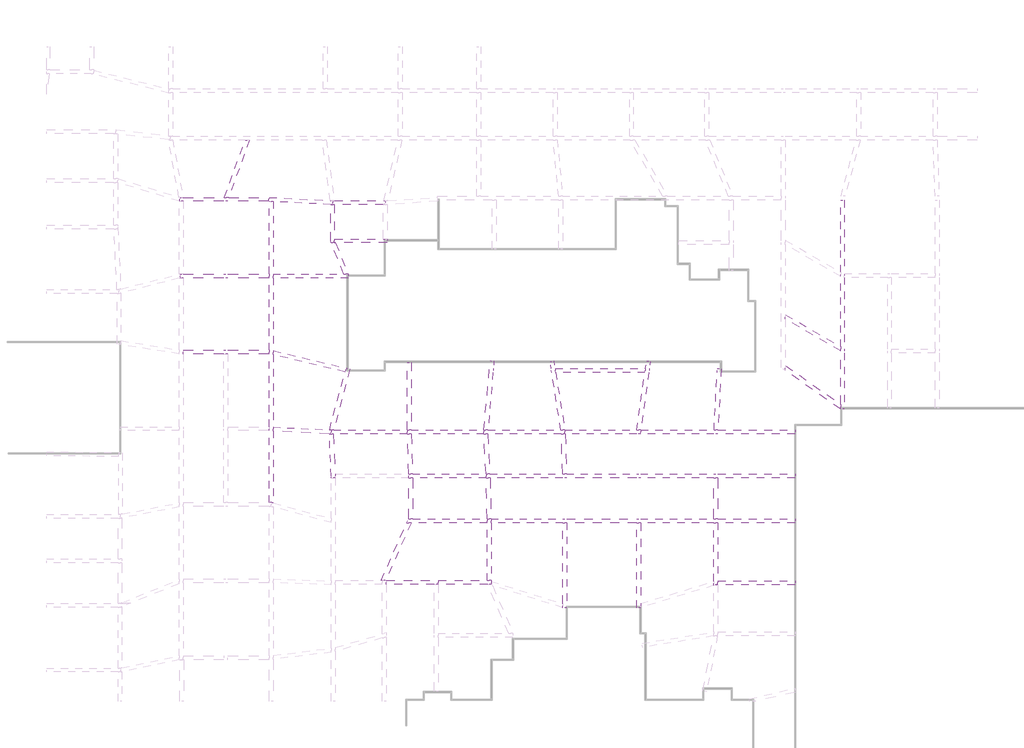
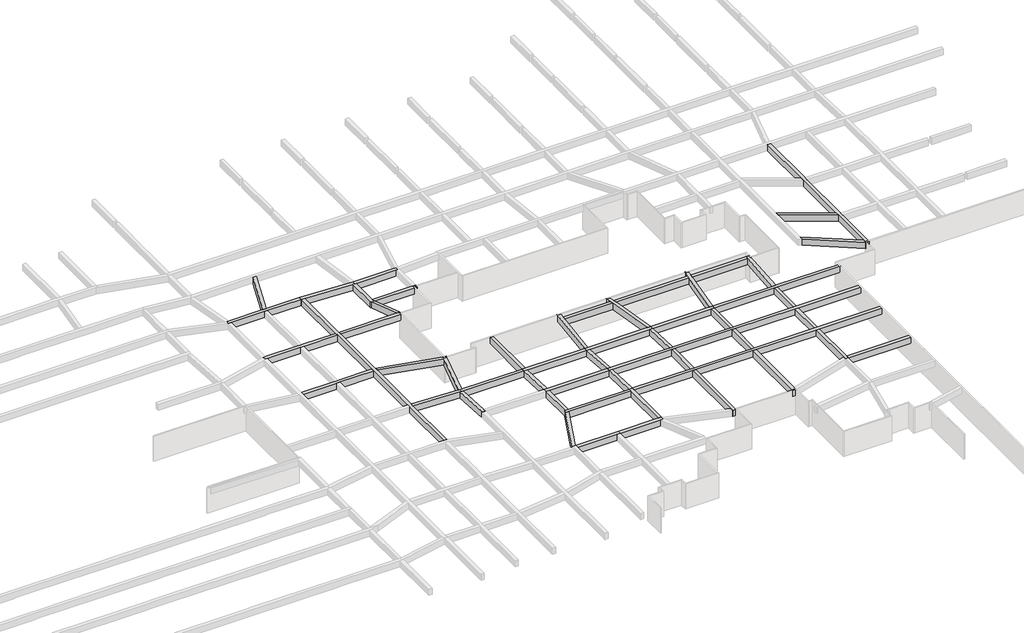
# One storey, part 17 of 45: 47 beams.
"""IFC4 building model written with IfcOpenShell, lengths in millimetres."""

from ifc_helpers import new_model, si_unit, frame, origin, place, context, project, spatial, polyline, outline, extrude, faceted_brep, element, save

model = new_model("IFC4")

# Units and contexts
model_context = context("Model", 3, world=origin())
ifc_project = project(units=[si_unit("LENGTHUNIT", "METRE", prefix="MILLI")], contexts=[model_context])

# Site, building, storey
site = spatial("IfcSite", under=ifc_project)
building = spatial("IfcBuilding", under=site)
storey = spatial("IfcBuildingStorey", under=building, Name="户型图", Elevation=0.0)

# Beams
placement = place(None, origin())
element("IfcBeam", 1, ObjectType="混凝土 - 矩形梁 : KL_beam", at=placement, inside=storey, context=model_context, shape_type="Brep", body=[
    faceted_brep([(-58675.077, -88790.3844516, 3300.0), (-58664.6026314, -88390.3844516, 3300.0), (-62792.0400184, -88390.3844516, 3300.0), (-63217.7111274, -88390.3844516, 3300.0), (-67462.9624722, -88390.3844516, 3300.0), (-67740.4118212, -88390.3844516, 3300.0), (-67799.2678102, -88790.3844516, 3300.0), (-67430.7823984, -88790.3844516, 3300.0), (-63277.6696197, -88790.3844516, 3300.0), (-62877.6696197, -88790.3844516, 3300.0), (-58675.077, -88790.3844516, 2500.0), (-67799.2678102, -88790.3844516, 2500.0), (-67430.7823984, -88790.3844516, 2500.0), (-63277.6696197, -88790.3844516, 2500.0), (-62877.6696197, -88790.3844516, 2500.0), (-58664.6026314, -88390.3844516, 2500.0), (-67740.4118212, -88390.3844516, 2500.0), (-67462.9624722, -88390.3844516, 2500.0), (-63217.7111274, -88390.3844516, 2500.0), (-62792.0400184, -88390.3844516, 2500.0)], [[[0, 1, 2, 3, 4, 5, 6, 7, 8, 9]], [[10, 0, 9, 8, 7, 6, 11, 12, 13, 14]], [[15, 10, 14, 13, 12, 11, 16, 17, 18, 19]], [[1, 15, 19, 18, 17, 16, 5, 4, 3, 2]], [[5, 16, 11, 6]], [[1, 0, 10, 15]]]),
])
element("IfcBeam", 2, ObjectType="混凝土 - 矩形梁 : KL_beam", at=placement, inside=storey, context=model_context, shape_type="Brep", body=[
    faceted_brep([(-67725.9320986, -96211.286122, 3300.0), (-67675.9190824, -96611.286122, 3300.0), (-67430.7823984, -96611.286122, 3300.0), (-63277.6696197, -96611.286122, 3300.0), (-62877.6696197, -96611.286122, 3300.0), (-58630.7823984, -96611.286122, 3300.0), (-58630.7823984, -96211.286122, 3300.0), (-62877.6696197, -96211.286122, 3300.0), (-63277.6696197, -96211.286122, 3300.0), (-67430.7823984, -96211.286122, 3300.0), (-67675.9190824, -96611.286122, 2500.0), (-67430.7823984, -96611.286122, 2500.0), (-63277.6696197, -96611.286122, 2500.0), (-62877.6696197, -96611.286122, 2500.0), (-58630.7823984, -96611.286122, 2500.0), (-67725.9320986, -96211.286122, 2500.0), (-67430.7823984, -96211.286122, 2500.0), (-63277.6696197, -96211.286122, 2500.0), (-62877.6696197, -96211.286122, 2500.0), (-58630.7823984, -96211.286122, 2500.0)], [[[0, 1, 2, 3, 4, 5, 6, 7, 8, 9]], [[1, 10, 11, 12, 13, 14, 5, 4, 3, 2]], [[10, 15, 16, 17, 18, 19, 14, 13, 12, 11]], [[15, 0, 9, 8, 7, 6, 19, 18, 17, 16]], [[0, 15, 10, 1]], [[6, 5, 14, 19]]]),
])
element("IfcBeam", 3, ObjectType="混凝土 - 矩形梁 : KL_beam", at=placement, inside=storey, context=model_context, shape_type="Brep", body=[
    faceted_brep([(-52173.5106555, -88730.5681671, 3300.0), (-52408.1333935, -88718.2721105, 3300.0), (-58664.6026314, -88390.3844516, 3300.0), (-58675.077, -88790.3844516, 3300.0), (-58630.7823984, -88792.7058333, 3300.0), (-58230.7823984, -88813.668945, 3300.0), (-52378.7478398, -89120.3610805, 3300.0), (-52183.9850241, -89130.5681671, 3300.0), (-58675.077, -88790.3844516, 2500.0), (-58630.7823984, -88792.7058333, 2500.0), (-58230.7823984, -88813.668945, 2500.0), (-52378.7478398, -89120.3610805, 2500.0), (-52183.9850241, -89130.5681671, 2500.0), (-58664.6026314, -88390.3844516, 2500.0), (-52408.1333935, -88718.2721105, 2500.0), (-52173.5106555, -88730.5681671, 2500.0)], [[[0, 1, 2, 3, 4, 5, 6, 7]], [[7, 6, 5, 4, 3, 8, 9, 10, 11, 12]], [[12, 11, 10, 9, 8, 13, 14, 15]], [[2, 1, 0, 15, 14, 13]], [[2, 13, 8, 3]], [[0, 7, 12, 15]]]),
])
element("IfcBeam", 4, ObjectType="混凝土 - 矩形梁 : KL_beam", at=placement, inside=storey, context=model_context, shape_type="Brep", body=[
    faceted_brep([(-46785.1341431, -88730.5681671, 3300.0), (-46937.8350231, -88730.5681671, 3300.0), (-52003.1410987, -88730.5681671, 3300.0), (-52173.5106555, -88730.5681671, 3300.0), (-52183.9850241, -89130.5681671, 3300.0), (-51978.7478398, -89130.5681671, 3300.0), (-46978.6472042, -89130.5681671, 3300.0), (-46772.3615365, -89130.5681671, 3300.0), (-52183.9850241, -89130.5681671, 2500.0), (-51978.7478398, -89130.5681671, 2500.0), (-46978.6472042, -89130.5681671, 2500.0), (-46772.3615365, -89130.5681671, 2500.0), (-52173.5106555, -88730.5681671, 2500.0), (-52003.1410987, -88730.5681671, 2500.0), (-46937.8350231, -88730.5681671, 2500.0), (-46785.1341431, -88730.5681671, 2500.0)], [[[0, 1, 2, 3, 4, 5, 6, 7]], [[7, 6, 5, 4, 8, 9, 10, 11]], [[11, 10, 9, 8, 12, 13, 14, 15]], [[3, 2, 1, 0, 15, 14, 13, 12]], [[3, 12, 8, 4]], [[0, 7, 11, 15]]]),
])
element("IfcBeam", 5, ObjectType="混凝土 - 矩形梁 : KL_beam", at=placement, inside=storey, context=model_context, shape_type="Brep", body=[
    faceted_brep([(-51978.7478398, -89130.5681671, 3300.0), (-52183.9850241, -89130.5681671, 3300.0), (-52355.5272319, -89121.578021, 3300.0), (-52378.7478398, -89120.3610805, 3300.0), (-52378.7478398, -92869.4623087, 3300.0), (-52313.6241975, -93030.5681671, 3300.0), (-51978.7478398, -93030.5681671, 3300.0), (-51978.7478398, -92630.5681671, 3300.0), (-52378.7478398, -89120.3610805, 2500.0), (-52378.7478398, -92869.4623087, 2500.0), (-52183.9850241, -89130.5681671, 2500.0), (-51978.7478398, -89130.5681671, 2500.0), (-51978.7478398, -92630.5681671, 2500.0), (-51978.7478398, -93030.5681671, 2500.0), (-52313.6241975, -93030.5681671, 2500.0), (-52355.5272319, -89121.578021, 2500.0)], [[[0, 1, 2, 3, 4, 5, 6, 7]], [[3, 8, 9, 4]], [[10, 11, 12, 13, 14, 9, 8, 15]], [[11, 0, 7, 6, 13, 12]], [[8, 3, 2, 1, 10, 15]], [[1, 0, 11, 10]], [[6, 5, 14, 13]], [[14, 5, 4, 9]]]),
])
element("IfcBeam", 6, ObjectType="混凝土 - 矩形梁 : KL_beam", at=placement, inside=storey, context=model_context, shape_type="Brep", body=[
    faceted_brep([(-46578.6472042, -93030.5681671, 3300.0), (-46578.6472042, -92630.5681671, 3300.0), (-46978.6472042, -92630.5681671, 3300.0), (-51978.7478398, -92630.5681671, 3300.0), (-51978.7478398, -93030.5681671, 3300.0), (-51882.1799262, -93030.5681671, 3300.0), (-46578.6472042, -93030.5681671, 2500.0), (-51978.7478398, -93030.5681671, 2500.0), (-51882.1799262, -93030.5681671, 2500.0), (-46578.6472042, -92630.5681671, 2500.0), (-51978.7478398, -92630.5681671, 2500.0), (-46978.6472042, -92630.5681671, 2500.0)], [[[0, 1, 2, 3, 4, 5]], [[6, 0, 5, 4, 7, 8]], [[9, 6, 8, 7, 10, 11]], [[1, 9, 11, 10, 3, 2]], [[4, 3, 10, 7]], [[1, 0, 6, 9]]]),
])
element("IfcBeam", 7, ObjectType="混凝土 - 矩形梁 : KL_beam", at=placement, inside=storey, context=model_context, shape_type="Brep", body=[
    faceted_brep([(-41387.6738698, -127942.8806028, 3300.0), (-41387.6738698, -127542.8806028, 3300.0), (-46687.6738698, -127542.8806028, 3300.0), (-46687.6738698, -127942.8806028, 3300.0), (-41787.6738698, -127942.8806028, 3300.0), (-41387.6738698, -127942.8806028, 2500.0), (-46687.6738698, -127942.8806028, 2500.0), (-41787.6738698, -127942.8806028, 2500.0), (-41387.6738698, -127542.8806028, 2500.0), (-46687.6738698, -127542.8806028, 2500.0)], [[[0, 1, 2, 3, 4]], [[5, 0, 4, 3, 6, 7]], [[8, 5, 7, 6, 9]], [[1, 8, 9, 2]], [[3, 2, 9, 6]], [[1, 0, 5, 8]]]),
])
element("IfcBeam", 8, ObjectType="混凝土 - 矩形梁 : KL_beam", at=placement, inside=storey, context=model_context, shape_type="Brep", body=[
    faceted_brep([(-35987.6738698, -127942.8806028, 3300.0), (-35987.6738698, -127702.1901429, 3300.0), (-35987.6738698, -127596.1274566, 3300.0), (-35987.6738698, -127542.8806028, 3300.0), (-36387.6738698, -127542.8806028, 3300.0), (-41387.6738698, -127542.8806028, 3300.0), (-41387.6738698, -127942.8806028, 3300.0), (-36320.0509821, -127942.8806028, 3300.0), (-35987.6738698, -127942.8806028, 2500.0), (-41387.6738698, -127942.8806028, 2500.0), (-36320.0509821, -127942.8806028, 2500.0), (-35987.6738698, -127542.8806028, 2500.0), (-35987.6738698, -127596.1274566, 2500.0), (-35987.6738698, -127702.1901429, 2500.0), (-41387.6738698, -127542.8806028, 2500.0), (-36387.6738698, -127542.8806028, 2500.0)], [[[0, 1, 2, 3, 4, 5, 6, 7]], [[8, 0, 7, 6, 9, 10]], [[11, 12, 13, 8, 10, 9, 14, 15]], [[3, 11, 15, 14, 5, 4]], [[3, 2, 1, 0, 8, 13, 12, 11]], [[6, 5, 14, 9]]]),
])
element("IfcBeam", 9, ObjectType="混凝土 - 矩形梁 : KL_beam", at=placement, inside=storey, context=model_context, shape_type="Brep", body=[
    faceted_brep([(-35987.6738698, -121242.8806028, 3300.0), (-35992.3975259, -121242.8806028, 3300.0), (-36387.6738698, -121242.8806028, 3300.0), (-36387.6738698, -121642.8806028, 3300.0), (-36387.6738698, -127542.8806028, 3300.0), (-35987.6738698, -127542.8806028, 3300.0), (-35987.6738698, -121642.8806028, 3300.0), (-35987.6738698, -121242.8806028, 2500.0), (-35987.6738698, -127542.8806028, 2500.0), (-35987.6738698, -121642.8806028, 2500.0), (-36387.6738698, -121242.8806028, 2500.0), (-35992.3975259, -121242.8806028, 2500.0), (-36387.6738698, -127542.8806028, 2500.0), (-36387.6738698, -121642.8806028, 2500.0)], [[[0, 1, 2, 3, 4, 5, 6]], [[7, 0, 6, 5, 8, 9]], [[10, 11, 7, 9, 8, 12, 13]], [[2, 10, 13, 12, 4, 3]], [[5, 4, 12, 8]], [[2, 1, 0, 7, 11, 10]]]),
])
element("IfcBeam", 10, ObjectType="混凝土 - 矩形梁 : KL_beam", at=placement, inside=storey, context=model_context, shape_type="Brep", body=[
    faceted_brep([(-44417.5553885, -121242.8806028, 3300.0), (-44595.6468626, -121642.8806028, 3300.0), (-44157.7923512, -121642.8806028, 3300.0), (-36387.6738698, -121642.8806028, 3300.0), (-36387.6738698, -121242.8806028, 3300.0), (-36392.5117893, -121242.8806028, 3300.0), (-43992.4702803, -121242.8806028, 3300.0), (-44392.4702803, -121242.8806028, 3300.0), (-44417.5553885, -121242.8806028, 2500.0), (-36387.6738698, -121242.8806028, 2500.0), (-36392.5117893, -121242.8806028, 2500.0), (-43992.4702803, -121242.8806028, 2500.0), (-44392.4702803, -121242.8806028, 2500.0), (-44595.6468626, -121642.8806028, 2500.0), (-36387.6738698, -121642.8806028, 2500.0), (-44157.7923512, -121642.8806028, 2500.0)], [[[0, 1, 2, 3, 4, 5, 6, 7]], [[8, 0, 7, 6, 5, 4, 9, 10, 11, 12]], [[13, 8, 12, 11, 10, 9, 14, 15]], [[1, 13, 15, 14, 3, 2]], [[4, 3, 14, 9]], [[1, 0, 8, 13]]]),
])
element("IfcBeam", 11, ObjectType="混凝土 - 矩形梁 : KL_beam", at=placement, inside=storey, context=model_context, shape_type="Brep", body=[
    faceted_brep([(-44157.7923512, -121642.8806028, 3300.0), (-44595.6468626, -121642.8806028, 3300.0), (-47222.4961059, -127542.8806028, 3300.0), (-47087.6738698, -127542.8806028, 3300.0), (-46784.6415945, -127542.8806028, 3300.0), (-44595.6468626, -121642.8806028, 2500.0), (-47222.4961059, -127542.8806028, 2500.0), (-44157.7923512, -121642.8806028, 2500.0), (-46784.6415945, -127542.8806028, 2500.0), (-47087.6738698, -127542.8806028, 2500.0)], [[[0, 1, 2, 3, 4]], [[1, 5, 6, 2]], [[5, 7, 8, 9, 6]], [[7, 0, 4, 8]], [[1, 0, 7, 5]], [[4, 3, 2, 6, 9, 8]]]),
])
element("IfcBeam", 12, ObjectType="混凝土 - 矩形梁 : KL_beam", at=placement, inside=storey, context=model_context, shape_type="Brep", body=[
    faceted_brep([(-4940.5977631, -121242.8806028, 3300.0), (-4940.5977631, -121642.8806028, 3300.0), (-4940.5977631, -121642.8806028, 2500.0), (-4940.5977631, -121242.8806028, 2500.0), (-12840.9657871, -121242.8806028, 3300.0), (-13240.9657871, -121242.8806028, 3300.0), (-20732.9657871, -121242.8806028, 3300.0), (-21132.9657871, -121242.8806028, 3300.0), (-28276.0008118, -121242.8806028, 3300.0), (-28676.0008118, -121242.8806028, 3300.0), (-35987.6738698, -121242.8806028, 3300.0), (-35987.6738698, -121642.8806028, 3300.0), (-28676.0008118, -121642.8806028, 3300.0), (-28276.0008118, -121642.8806028, 3300.0), (-21132.9657871, -121642.8806028, 3300.0), (-20732.9657871, -121642.8806028, 3300.0), (-13240.9657871, -121642.8806028, 3300.0), (-12840.9657871, -121642.8806028, 3300.0), (-35987.6738698, -121642.8806028, 2500.0), (-28676.0008118, -121642.8806028, 2500.0), (-28276.0008118, -121642.8806028, 2500.0), (-21132.9657871, -121642.8806028, 2500.0), (-20732.9657871, -121642.8806028, 2500.0), (-13240.9657871, -121642.8806028, 2500.0), (-12840.9657871, -121642.8806028, 2500.0), (-35987.6738698, -121242.8806028, 2500.0), (-28676.0008118, -121242.8806028, 2500.0), (-28276.0008118, -121242.8806028, 2500.0), (-21132.9657871, -121242.8806028, 2500.0), (-20732.9657871, -121242.8806028, 2500.0), (-13240.9657871, -121242.8806028, 2500.0), (-12840.9657871, -121242.8806028, 2500.0)], [[[0, 1, 2, 3]], [[1, 0, 4, 5, 6, 7, 8, 9, 10, 11, 12, 13, 14, 15, 16, 17]], [[2, 1, 17, 16, 15, 14, 13, 12, 11, 18, 19, 20, 21, 22, 23, 24]], [[3, 2, 24, 23, 22, 21, 20, 19, 18, 25, 26, 27, 28, 29, 30, 31]], [[0, 3, 31, 30, 29, 28, 27, 26, 25, 10, 9, 8, 7, 6, 5, 4]], [[11, 10, 25, 18]]]),
])
element("IfcBeam", 13, ObjectType="混凝土 - 矩形梁 : KL_beam", at=placement, inside=storey, context=model_context, shape_type="Brep", body=[
    faceted_brep([(-28462.3909606, -112558.1512167, 3300.0), (-28462.3909606, -112158.1512167, 3300.0), (-28867.3770109, -112158.1512167, 3300.0), (-36315.5397573, -112158.1512167, 3300.0), (-36717.0676923, -112158.1512167, 3300.0), (-36717.0676923, -112558.1512167, 3300.0), (-36322.6397923, -112558.1512167, 3300.0), (-28826.6420326, -112558.1512167, 3300.0), (-28462.3909606, -112558.1512167, 2500.0), (-36717.0676923, -112558.1512167, 2500.0), (-36322.6397923, -112558.1512167, 2500.0), (-28826.6420326, -112558.1512167, 2500.0), (-28462.3909606, -112158.1512167, 2500.0), (-36717.0676923, -112158.1512167, 2500.0), (-36315.5397573, -112158.1512167, 2500.0), (-28867.3770109, -112158.1512167, 2500.0)], [[[0, 1, 2, 3, 4, 5, 6, 7]], [[8, 0, 7, 6, 5, 9, 10, 11]], [[12, 8, 11, 10, 9, 13, 14, 15]], [[1, 12, 15, 14, 13, 4, 3, 2]], [[1, 0, 8, 12]], [[4, 13, 9, 5]]]),
])
element("IfcBeam", 14, ObjectType="混凝土 - 矩形梁 : KL_beam", at=placement, inside=storey, context=model_context, shape_type="Brep", body=[
    faceted_brep([(-20759.5525702, -112558.1512167, 3300.0), (-20703.3362363, -112158.1512167, 3300.0), (-21107.2672653, -112158.1512167, 3300.0), (-28462.3909606, -112158.1512167, 3300.0), (-28462.3909606, -112558.1512167, 3300.0), (-28426.3982149, -112558.1512167, 3300.0), (-21132.9657871, -112558.1512167, 3300.0), (-20759.5525702, -112558.1512167, 2500.0), (-28462.3909606, -112558.1512167, 2500.0), (-28426.3982149, -112558.1512167, 2500.0), (-21132.9657871, -112558.1512167, 2500.0), (-20703.3362363, -112158.1512167, 2500.0), (-28462.3909606, -112158.1512167, 2500.0), (-21107.2672653, -112158.1512167, 2500.0)], [[[0, 1, 2, 3, 4, 5, 6]], [[7, 0, 6, 5, 4, 8, 9, 10]], [[11, 7, 10, 9, 8, 12, 13]], [[1, 11, 13, 12, 3, 2]], [[4, 3, 12, 8]], [[1, 0, 7, 11]]]),
])
element("IfcBeam", 15, ObjectType="混凝土 - 矩形梁 : KL_beam", at=placement, inside=storey, context=model_context, shape_type="Brep", body=[
    faceted_brep([(-4940.9657871, -112158.1512167, 3300.0), (-4940.9657871, -112558.1512167, 3300.0), (-4940.9657871, -112558.1512167, 2500.0), (-4940.9657871, -112158.1512167, 2500.0), (-12830.2097621, -112158.1512167, 3300.0), (-13230.7587005, -112158.1512167, 3300.0), (-20703.3362363, -112158.1512167, 3300.0), (-20759.5525702, -112558.1512167, 3300.0), (-20732.9657871, -112558.1512167, 3300.0), (-13240.9657871, -112558.1512167, 3300.0), (-12840.9657871, -112558.1512167, 3300.0), (-20759.5525702, -112558.1512167, 2500.0), (-20732.9657871, -112558.1512167, 2500.0), (-13240.9657871, -112558.1512167, 2500.0), (-12840.9657871, -112558.1512167, 2500.0), (-20703.3362363, -112158.1512167, 2500.0), (-13230.7587005, -112158.1512167, 2500.0), (-12830.2097621, -112158.1512167, 2500.0)], [[[0, 1, 2, 3]], [[1, 0, 4, 5, 6, 7, 8, 9, 10]], [[2, 1, 10, 9, 8, 7, 11, 12, 13, 14]], [[3, 2, 14, 13, 12, 11, 15, 16, 17]], [[0, 3, 17, 16, 15, 6, 5, 4]], [[7, 6, 15, 11]]]),
])
element("IfcBeam", 16, ObjectType="混凝土 - 矩形梁 : KL_beam", at=placement, inside=storey, context=model_context, shape_type="Brep", body=[
    faceted_brep([(-4940.771094, -116668.4603553, 3300.0), (-4940.771094, -117068.4603553, 3300.0), (-4940.771094, -117068.4603553, 2500.0), (-4940.771094, -116668.4603553, 2500.0), (-12840.9657871, -116668.4603553, 3300.0), (-13240.9657871, -116668.4603553, 3300.0), (-20732.9657871, -116668.4603553, 3300.0), (-21132.9657871, -116668.4603553, 3300.0), (-28282.8630569, -116668.4603553, 3300.0), (-28683.1068746, -116668.4603553, 3300.0), (-36107.2276182, -116668.4603553, 3300.0), (-36507.7765566, -116668.4603553, 3300.0), (-36486.8134449, -117068.4603553, 3300.0), (-36092.1826121, -117068.4603553, 3300.0), (-28676.0008118, -117068.4603553, 3300.0), (-28276.0008118, -117068.4603553, 3300.0), (-21132.9657871, -117068.4603553, 3300.0), (-20732.9657871, -117068.4603553, 3300.0), (-13240.9657871, -117068.4603553, 3300.0), (-12840.9657871, -117068.4603553, 3300.0), (-36486.8134449, -117068.4603553, 2500.0), (-36092.1826121, -117068.4603553, 2500.0), (-28676.0008118, -117068.4603553, 2500.0), (-28276.0008118, -117068.4603553, 2500.0), (-21132.9657871, -117068.4603553, 2500.0), (-20732.9657871, -117068.4603553, 2500.0), (-13240.9657871, -117068.4603553, 2500.0), (-12840.9657871, -117068.4603553, 2500.0), (-36507.7765566, -116668.4603553, 2500.0), (-36107.2276182, -116668.4603553, 2500.0), (-28683.1068746, -116668.4603553, 2500.0), (-28282.8630569, -116668.4603553, 2500.0), (-21132.9657871, -116668.4603553, 2500.0), (-20732.9657871, -116668.4603553, 2500.0), (-13240.9657871, -116668.4603553, 2500.0), (-12840.9657871, -116668.4603553, 2500.0)], [[[0, 1, 2, 3]], [[1, 0, 4, 5, 6, 7, 8, 9, 10, 11, 12, 13, 14, 15, 16, 17, 18, 19]], [[2, 1, 19, 18, 17, 16, 15, 14, 13, 12, 20, 21, 22, 23, 24, 25, 26, 27]], [[3, 2, 27, 26, 25, 24, 23, 22, 21, 20, 28, 29, 30, 31, 32, 33, 34, 35]], [[0, 3, 35, 34, 33, 32, 31, 30, 29, 28, 11, 10, 9, 8, 7, 6, 5, 4]], [[12, 11, 28, 20]]]),
])
element("IfcBeam", 17, ObjectType="混凝土 - 矩形梁 : KL_beam", at=placement, inside=storey, context=model_context, shape_type="Brep", body=[
    faceted_brep([(-44543.1279322, -112158.1512167, 3300.0), (-44543.1279322, -112558.1512167, 3300.0), (-44142.8841144, -112558.1512167, 3300.0), (-36723.1887307, -112558.1512167, 3300.0), (-36717.0676923, -112558.1512167, 3300.0), (-36717.0676923, -112158.1512167, 3300.0), (-44150.3958174, -112158.1512167, 3300.0), (-44543.1279322, -112558.1512167, 2500.0), (-44142.8841144, -112558.1512167, 2500.0), (-36723.1887307, -112558.1512167, 2500.0), (-36717.0676923, -112558.1512167, 2500.0), (-44543.1279322, -112158.1512167, 2500.0), (-44150.3958174, -112158.1512167, 2500.0), (-36717.0676923, -112158.1512167, 2500.0)], [[[0, 1, 2, 3, 4, 5, 6]], [[1, 7, 8, 9, 10, 4, 3, 2]], [[7, 11, 12, 13, 10, 9, 8]], [[11, 0, 6, 5, 13, 12]], [[5, 4, 10, 13]], [[0, 11, 7, 1]]]),
])
element("IfcBeam", 18, ObjectType="混凝土 - 矩形梁 : KL_beam", at=placement, inside=storey, context=model_context, shape_type="Brep", body=[
    faceted_brep([(-44399.5927742, -116668.4603553, 3300.0), (-44385.6244664, -117068.4603553, 3300.0), (-43992.4702803, -117068.4603553, 3300.0), (-36492.2968754, -117068.4603553, 3300.0), (-36486.8134449, -117068.4603553, 3300.0), (-36507.7765566, -116668.4603553, 3300.0), (-43999.3489565, -116668.4603553, 3300.0), (-44399.5927742, -116668.4603553, 2500.0), (-36507.7765566, -116668.4603553, 2500.0), (-43999.3489565, -116668.4603553, 2500.0), (-44385.6244664, -117068.4603553, 2500.0), (-36486.8134449, -117068.4603553, 2500.0), (-36492.2968754, -117068.4603553, 2500.0), (-43992.4702803, -117068.4603553, 2500.0)], [[[0, 1, 2, 3, 4, 5, 6]], [[7, 0, 6, 5, 8, 9]], [[10, 7, 9, 8, 11, 12, 13]], [[1, 10, 13, 12, 11, 4, 3, 2]], [[1, 0, 7, 10]], [[5, 4, 11, 8]]]),
])
element("IfcBeam", 19, ObjectType="混凝土 - 矩形梁 : KL_beam", at=placement, inside=storey, context=model_context, shape_type="Brep", body=[
    faceted_brep([(-52328.3755535, -112158.1512167, 3300.0), (-52338.8499222, -112558.1512167, 3300.0), (-52122.8567128, -112558.1512167, 3300.0), (-44543.1279322, -112558.1512167, 3300.0), (-44557.09624, -112158.1512167, 3300.0), (-52072.656383, -112158.1512167, 3300.0), (-52328.3755535, -112158.1512167, 2500.0), (-44557.09624, -112158.1512167, 2500.0), (-52072.656383, -112158.1512167, 2500.0), (-52338.8499222, -112558.1512167, 2500.0), (-44543.1279322, -112558.1512167, 2500.0), (-52122.8567128, -112558.1512167, 2500.0)], [[[0, 1, 2, 3, 4, 5]], [[6, 0, 5, 4, 7, 8]], [[9, 6, 8, 7, 10, 11]], [[1, 9, 11, 10, 3, 2]], [[1, 0, 6, 9]], [[4, 3, 10, 7]]]),
])
element("IfcBeam", 20, ObjectType="混凝土 - 矩形梁 : KL_beam", at=placement, inside=storey, context=model_context, shape_type="Brep", body=[
    faceted_brep([(-52338.8499222, -112558.1512167, 3300.0), (-52328.3755535, -112158.1512167, 3300.0), (-52484.5734274, -112149.965233, 3300.0), (-58230.7823984, -111848.8191815, 3300.0), (-58230.7823984, -112249.3681199, 3300.0), (-52523.9139435, -112548.4524223, 3300.0), (-52328.3755535, -112158.1512167, 2500.0), (-52484.5734274, -112149.965233, 2500.0), (-58230.7823984, -111848.8191815, 2500.0), (-52338.8499222, -112558.1512167, 2500.0), (-52523.9139435, -112548.4524223, 2500.0), (-58230.7823984, -112249.3681199, 2500.0)], [[[0, 1, 2, 3, 4, 5]], [[1, 6, 7, 8, 3, 2]], [[6, 9, 10, 11, 8, 7]], [[9, 0, 5, 4, 11, 10]], [[0, 9, 6, 1]], [[4, 3, 8, 11]]]),
])
element("IfcBeam", 21, ObjectType="混凝土 - 矩形梁 : KL_beam", at=placement, inside=storey, context=model_context, shape_type="Brep", body=[
    faceted_brep([(-52122.8567128, -112558.1512167, 3300.0), (-52338.8499222, -112558.1512167, 3300.0), (-52523.9139435, -112548.4524223, 3300.0), (-52297.3620817, -116871.3194631, 3300.0), (-52287.0303654, -117068.4603553, 3300.0), (-51897.3620817, -117068.4603553, 3300.0), (-51886.481427, -117068.4603553, 3300.0), (-51907.4445387, -116668.4603553, 3300.0), (-52287.0303654, -117068.4603553, 2500.0), (-52523.9139435, -112548.4524223, 2500.0), (-52297.3620817, -116871.3194631, 2500.0), (-52338.8499222, -112558.1512167, 2500.0), (-52122.8567128, -112558.1512167, 2500.0), (-51907.4445387, -116668.4603553, 2500.0), (-51886.481427, -117068.4603553, 2500.0), (-51897.3620817, -117068.4603553, 2500.0)], [[[0, 1, 2, 3, 4, 5, 6, 7]], [[8, 4, 3, 2, 9, 10]], [[11, 12, 13, 14, 15, 8, 10, 9]], [[12, 0, 7, 6, 14, 13]], [[1, 0, 12, 11]], [[2, 1, 11, 9]], [[6, 5, 4, 8, 15, 14]]]),
])
element("IfcBeam", 22, ObjectType="混凝土 - 矩形梁 : KL_beam", at=placement, inside=storey, context=model_context, shape_type="Brep", body=[
    faceted_brep([(-44142.8841144, -112558.1512167, 3300.0), (-44543.1279322, -112558.1512167, 3300.0), (-44399.5927742, -116668.4603553, 3300.0), (-43999.3489565, -116668.4603553, 3300.0), (-44142.8841144, -112558.1512167, 2500.0), (-43999.3489565, -116668.4603553, 2500.0), (-44543.1279322, -112558.1512167, 2500.0), (-44399.5927742, -116668.4603553, 2500.0), (-44557.09624, -112158.1512167, 3300.0), (-44557.09624, -112158.1512167, 2500.0), (-44550.3958174, -112158.1512167, 3300.0), (-44543.1279322, -112158.1512167, 3300.0), (-44543.1279322, -112158.1512167, 2500.0), (-44550.3958174, -112158.1512167, 2500.0)], [[[0, 1, 2, 3]], [[4, 0, 3, 5]], [[6, 4, 5, 7]], [[8, 9, 6, 7, 2, 1]], [[9, 8, 10, 11, 12, 13]], [[6, 1, 0, 4]], [[1, 6, 12, 11]], [[11, 10, 8, 1]], [[9, 13, 12, 6]], [[3, 2, 7, 5]]]),
])
element("IfcBeam", 23, ObjectType="混凝土 - 矩形梁 : KL_beam", at=placement, inside=storey, context=model_context, shape_type="Brep", body=[
    faceted_brep([(-43992.4702803, -117068.4603553, 3300.0), (-44385.6244664, -117068.4603553, 3300.0), (-44392.4702803, -117068.4603553, 3300.0), (-44392.4702803, -121242.8806028, 3300.0), (-43992.4702803, -121242.8806028, 3300.0), (-44392.4702803, -121242.8806028, 2500.0), (-44392.4702803, -117068.4603553, 2500.0), (-44385.6244664, -117068.4603553, 2500.0), (-43992.4702803, -117068.4603553, 2500.0), (-43992.4702803, -121242.8806028, 2500.0)], [[[0, 1, 2, 3, 4]], [[5, 3, 2, 6]], [[6, 7, 8, 9, 5]], [[8, 0, 4, 9]], [[0, 8, 7, 6, 2, 1]], [[4, 3, 5, 9]]]),
])
element("IfcBeam", 24, ObjectType="混凝土 - 矩形梁 : KL_beam", at=placement, inside=storey, context=model_context, shape_type="Brep", body=[
    faceted_brep([(-58630.7823984, -119570.4077047, 3300.0), (-58404.4518989, -119570.4077047, 3300.0), (-58230.7823984, -119616.9423071, 3300.0), (-58230.7823984, -112249.3681199, 3300.0), (-58230.7823984, -111848.8191815, 3300.0), (-58230.7823984, -104465.0874486, 3300.0), (-58230.7823984, -104053.6825329, 3300.0), (-58230.7823984, -96611.286122, 3300.0), (-58230.7823984, -96211.286122, 3300.0), (-58230.7823984, -88813.668945, 3300.0), (-58630.7823984, -88792.7058333, 3300.0), (-58630.7823984, -96211.286122, 3300.0), (-58630.7823984, -96611.286122, 3300.0), (-58630.7823984, -104011.286122, 3300.0), (-58630.7823984, -104411.286122, 3300.0), (-58630.7823984, -111828.4346923, 3300.0), (-58630.7823984, -112228.4346923, 3300.0), (-58230.7823984, -119616.9423071, 2500.0), (-58230.7823984, -112249.3681199, 2500.0), (-58230.7823984, -111848.8191815, 2500.0), (-58230.7823984, -104465.0874486, 2500.0), (-58230.7823984, -104053.6825329, 2500.0), (-58230.7823984, -96611.286122, 2500.0), (-58230.7823984, -96211.286122, 2500.0), (-58230.7823984, -88813.668945, 2500.0), (-58404.4518989, -119570.4077047, 2500.0), (-58630.7823984, -119570.4077047, 2500.0), (-58630.7823984, -112228.4346923, 2500.0), (-58630.7823984, -111828.4346923, 2500.0), (-58630.7823984, -104411.286122, 2500.0), (-58630.7823984, -104011.286122, 2500.0), (-58630.7823984, -96611.286122, 2500.0), (-58630.7823984, -96211.286122, 2500.0), (-58630.7823984, -88792.7058333, 2500.0)], [[[0, 1, 2, 3, 4, 5, 6, 7, 8, 9, 10, 11, 12, 13, 14, 15, 16]], [[2, 17, 18, 19, 20, 21, 22, 23, 24, 9, 8, 7, 6, 5, 4, 3]], [[25, 26, 27, 28, 29, 30, 31, 32, 33, 24, 23, 22, 21, 20, 19, 18, 17]], [[26, 0, 16, 15, 14, 13, 12, 11, 10, 33, 32, 31, 30, 29, 28, 27]], [[1, 0, 26, 25]], [[2, 1, 25, 17]], [[10, 9, 24, 33]]]),
])
element("IfcBeam", 25, ObjectType="混凝土 - 矩形梁 : KL_beam", at=placement, inside=storey, context=model_context, shape_type="Brep", body=[
    faceted_brep([(-50596.4418387, -96611.286122, 3300.0), (-50596.4418387, -96211.286122, 3300.0), (-51027.88611, -96211.286122, 3300.0), (-58230.7823984, -96211.286122, 3300.0), (-58230.7823984, -96611.286122, 3300.0), (-50596.4418387, -96611.286122, 2500.0), (-58230.7823984, -96611.286122, 2500.0), (-50596.4418387, -96211.286122, 2500.0), (-58230.7823984, -96211.286122, 2500.0), (-51027.88611, -96211.286122, 2500.0)], [[[0, 1, 2, 3, 4]], [[5, 0, 4, 6]], [[7, 5, 6, 8, 9]], [[1, 7, 9, 8, 3, 2]], [[4, 3, 8, 6]], [[1, 0, 5, 7]]]),
])
element("IfcBeam", 26, ObjectType="混凝土 - 矩形梁 : KL_beam", at=placement, inside=storey, context=model_context, shape_type="Brep", body=[
    faceted_brep([(-50596.4418387, -96211.286122, 3300.0), (-51882.1799262, -93030.5681671, 3300.0), (-51978.7478398, -93030.5681671, 3300.0), (-52313.6241975, -93030.5681671, 3300.0), (-51027.88611, -96211.286122, 3300.0), (-52313.6241975, -93030.5681671, 2500.0), (-51027.88611, -96211.286122, 2500.0), (-51882.1799262, -93030.5681671, 2500.0), (-50596.4418387, -96211.286122, 2500.0), (-51978.7478398, -93030.5681671, 2500.0)], [[[0, 1, 2, 3, 4]], [[3, 5, 6, 4]], [[7, 8, 6, 5, 9]], [[1, 0, 8, 7]], [[5, 3, 2, 1, 7, 9]], [[0, 4, 6, 8]]]),
])
element("IfcBeam", 27, ObjectType="混凝土 - 矩形梁 : KL_beam", at=placement, inside=storey, context=model_context, shape_type="Brep", body=[
    faceted_brep([(-67430.7823984, -104011.286122, 3300.0), (-67430.7823984, -104411.286122, 3300.0), (-63277.6696197, -104411.286122, 3300.0), (-62877.6696197, -104411.286122, 3300.0), (-58630.7823984, -104411.286122, 3300.0), (-58630.7823984, -104011.286122, 3300.0), (-62877.6696197, -104011.286122, 3300.0), (-63277.6696197, -104011.286122, 3300.0), (-67430.7823984, -104411.286122, 2500.0), (-63277.6696197, -104411.286122, 2500.0), (-62877.6696197, -104411.286122, 2500.0), (-58630.7823984, -104411.286122, 2500.0), (-67430.7823984, -104011.286122, 2500.0), (-63277.6696197, -104011.286122, 2500.0), (-62877.6696197, -104011.286122, 2500.0), (-58630.7823984, -104011.286122, 2500.0)], [[[0, 1, 2, 3, 4, 5, 6, 7]], [[1, 8, 9, 10, 11, 4, 3, 2]], [[8, 12, 13, 14, 15, 11, 10, 9]], [[12, 0, 7, 6, 5, 15, 14, 13]], [[1, 0, 12, 8]], [[5, 4, 11, 15]]]),
])
element("IfcBeam", 28, ObjectType="混凝土 - 矩形梁 : KL_beam", at=placement, inside=storey, context=model_context, shape_type="Brep", body=[
    faceted_brep([(-310.8072722, -110031.7719732, 3300.0), (89.1927278, -110031.7719732, 3300.0), (89.1927278, -104288.0123265, 3300.0), (89.1927278, -103888.0123265, 3300.0), (89.1927278, -96568.0123265, 3300.0), (89.1927278, -96168.0123265, 3300.0), (89.1927278, -88687.9389906, 3300.0), (-310.8072722, -88687.9389906, 3300.0), (-310.8072722, -96021.0575371, 3300.0), (-310.8072722, -96483.1397428, 3300.0), (-310.8072722, -103641.0575371, 3300.0), (-310.8072722, -104103.1397428, 3300.0), (-310.8072722, -109542.6055214, 3300.0), (-310.8072722, -110031.7719732, 2500.0), (-310.8072722, -88687.9389906, 2500.0), (-310.8072722, -96021.0575371, 2500.0), (-310.8072722, -96483.1397428, 2500.0), (-310.8072722, -103641.0575371, 2500.0), (-310.8072722, -104103.1397428, 2500.0), (-310.8072722, -109542.6055214, 2500.0), (89.1927278, -110031.7719732, 2500.0), (89.1927278, -88687.9389906, 2500.0), (89.1927278, -96168.0123265, 2500.0), (89.1927278, -96568.0123265, 2500.0), (89.1927278, -103888.0123265, 2500.0), (89.1927278, -104288.0123265, 2500.0)], [[[0, 1, 2, 3, 4, 5, 6, 7, 8, 9, 10, 11, 12]], [[13, 0, 12, 11, 10, 9, 8, 7, 14, 15, 16, 17, 18, 19]], [[20, 13, 19, 18, 17, 16, 15, 14, 21, 22, 23, 24, 25]], [[1, 20, 25, 24, 23, 22, 21, 6, 5, 4, 3, 2]], [[7, 6, 21, 14]], [[1, 0, 13, 20]]]),
])
element("IfcBeam", 29, ObjectType="混凝土 - 矩形梁 : KL_beam", at=placement, inside=storey, context=model_context, shape_type="SweptSolid", body=[
    extrude(outline(polyline([(-5961.9880078, -100834.7253412), (-5961.9880078, -100372.6431355), (-310.8072722, -103641.0575371), (-310.8072722, -104103.1397428), (-5961.9880078, -100834.7253412)])), frame((0.0, 0.0, 2500.0), z_axis=(0.0, 0.0, 1.0), x_axis=(1.0, 0.0, 0.0)), (0.0, 0.0, 1.0), 800.0),
])
element("IfcBeam", 30, ObjectType="混凝土 - 矩形梁 : KL_beam", at=placement, inside=storey, context=model_context, shape_type="SweptSolid", body=[
    extrude(outline(polyline([(-310.8072722, -110031.7719732), (-5961.9880078, -106053.71057), (-5961.9880078, -105564.5441182), (-310.8072722, -109542.6055214), (-310.8072722, -110031.7719732)])), frame((0.0, 0.0, 2500.0), z_axis=(0.0, 0.0, 1.0), x_axis=(1.0, 0.0, 0.0)), (0.0, 0.0, 1.0), 800.0),
])
element("IfcBeam", 31, ObjectType="混凝土 - 矩形梁 : KL_beam", at=placement, inside=storey, context=model_context, shape_type="Brep", body=[
    faceted_brep([(-36096.8034751, -105068.4987721, 3300.0), (-35698.3255959, -105103.3610692, 3300.0), (-35698.3255959, -105103.3610692, 2500.0), (-36096.8034751, -105068.4987721, 2500.0), (-36717.0676923, -112158.1512167, 3300.0), (-36315.5397573, -112158.1512167, 3300.0), (-35801.4540434, -106282.1246187, 3300.0), (-35766.458578, -105882.1246187, 3300.0), (-36315.5397573, -112158.1512167, 2500.0), (-35801.4540434, -106282.1246187, 2500.0), (-35766.458578, -105882.1246187, 2500.0), (-36717.0676923, -112158.1512167, 2500.0)], [[[0, 1, 2, 3]], [[1, 0, 4, 5, 6, 7]], [[2, 1, 7, 6, 5, 8, 9, 10]], [[3, 2, 10, 9, 8, 11]], [[0, 3, 11, 4]], [[5, 4, 11, 8]]]),
])
element("IfcBeam", 32, ObjectType="混凝土 - 矩形梁 : KL_beam", at=placement, inside=storey, context=model_context, shape_type="Brep", body=[
    faceted_brep([(-29972.7163606, -105179.3132233, 3300.0), (-29577.6410244, -105116.7394373, 3300.0), (-29577.6410244, -105116.7394373, 2500.0), (-29972.7163606, -105179.3132233, 2500.0), (-29861.4019711, -105882.1246187, 3300.0), (-29798.048195, -106282.1246187, 3300.0), (-28867.3770109, -112158.1512167, 3300.0), (-28462.3909606, -112158.1512167, 3300.0), (-29393.0621447, -106282.1246187, 3300.0), (-29456.4159208, -105882.1246187, 3300.0), (-28462.3909606, -112158.1512167, 2500.0), (-29393.0621447, -106282.1246187, 2500.0), (-29456.4159208, -105882.1246187, 2500.0), (-28867.3770109, -112158.1512167, 2500.0), (-29798.048195, -106282.1246187, 2500.0), (-29861.4019711, -105882.1246187, 2500.0)], [[[0, 1, 2, 3]], [[1, 0, 4, 5, 6, 7, 8, 9]], [[2, 1, 9, 8, 7, 10, 11, 12]], [[3, 2, 12, 11, 10, 13, 14, 15]], [[0, 3, 15, 14, 13, 6, 5, 4]], [[7, 6, 13, 10]]]),
])
element("IfcBeam", 33, ObjectType="混凝土 - 矩形梁 : KL_beam", at=placement, inside=storey, context=model_context, shape_type="Brep", body=[
    faceted_brep([(-20115.4998945, -105101.3596947, 3300.0), (-19719.392667, -105157.0289351, 3300.0), (-19719.392667, -105157.0289351, 2500.0), (-20115.4998945, -105101.3596947, 2500.0), (-20225.2292486, -105882.1246187, 3300.0), (-20281.4455825, -106282.1246187, 3300.0), (-21107.2672653, -112158.1512167, 3300.0), (-20703.3362363, -112158.1512167, 3300.0), (-19877.5145535, -106282.1246187, 3300.0), (-19821.2982196, -105882.1246187, 3300.0), (-20703.3362363, -112158.1512167, 2500.0), (-19877.5145535, -106282.1246187, 2500.0), (-19821.2982196, -105882.1246187, 2500.0), (-21107.2672653, -112158.1512167, 2500.0), (-20281.4455825, -106282.1246187, 2500.0), (-20225.2292486, -105882.1246187, 2500.0)], [[[0, 1, 2, 3]], [[1, 0, 4, 5, 6, 7, 8, 9]], [[2, 1, 9, 8, 7, 10, 11, 12]], [[3, 2, 12, 11, 10, 13, 14, 15]], [[0, 3, 15, 14, 13, 6, 5, 4]], [[7, 6, 13, 10]]]),
])
element("IfcBeam", 34, ObjectType="混凝土 - 矩形梁 : KL_beam", at=placement, inside=storey, context=model_context, shape_type="Brep", body=[
    faceted_brep([(-12502.3942698, -105903.0590012, 3300.0), (-12901.8460837, -105882.1246187, 3300.0), (-12922.8091954, -106282.1246187, 3300.0), (-13230.7587005, -112158.1512167, 3300.0), (-12830.2097621, -112158.1512167, 3300.0), (-12502.3942698, -105903.0590012, 2500.0), (-12830.2097621, -112158.1512167, 2500.0), (-12901.8460837, -105882.1246187, 2500.0), (-13230.7587005, -112158.1512167, 2500.0), (-12922.8091954, -106282.1246187, 2500.0)], [[[0, 1, 2, 3, 4]], [[5, 0, 4, 6]], [[7, 5, 6, 8, 9]], [[1, 7, 9, 8, 3, 2]], [[4, 3, 8, 6]], [[1, 0, 5, 7]]]),
])
element("IfcBeam", 35, ObjectType="混凝土 - 矩形梁 : KL_beam", at=placement, inside=storey, context=model_context, shape_type="Brep", body=[
    faceted_brep([(-35766.458578, -105882.1246187, 3300.0), (-35801.4540434, -106282.1246187, 3300.0), (-29798.048195, -106282.1246187, 3300.0), (-29861.4019711, -105882.1246187, 3300.0), (-35801.4540434, -106282.1246187, 2500.0), (-29798.048195, -106282.1246187, 2500.0), (-35766.458578, -105882.1246187, 2500.0), (-29861.4019711, -105882.1246187, 2500.0)], [[[0, 1, 2, 3]], [[1, 4, 5, 2]], [[4, 6, 7, 5]], [[6, 0, 3, 7]], [[1, 0, 6, 4]], [[3, 2, 5, 7]]]),
    faceted_brep([(-12501.2971453, -105882.1246187, 2500.0), (-12501.2971453, -105882.1246187, 3300.0), (-12502.3942698, -105903.0590012, 3300.0), (-12502.3942698, -105903.0590012, 2500.0), (-12901.8460837, -105882.1246187, 2500.0), (-12901.8460837, -105882.1246187, 3300.0), (-12922.8091954, -106282.1246187, 3300.0), (-12922.8091954, -106282.1246187, 2500.0), (-19821.2982196, -105882.1246187, 3300.0), (-19877.5145535, -106282.1246187, 3300.0), (-19877.5145535, -106282.1246187, 2500.0), (-19821.2982196, -105882.1246187, 2500.0)], [[[0, 1, 2, 3]], [[4, 5, 6, 7]], [[5, 4, 3, 2]], [[2, 1, 5]], [[0, 3, 4]], [[6, 5, 8, 9]], [[7, 6, 9, 10]], [[4, 7, 10, 11]], [[1, 0, 4, 11, 8, 5]], [[9, 8, 11, 10]]]),
    faceted_brep([(-29393.0621447, -106282.1246187, 3300.0), (-29456.4159208, -105882.1246187, 3300.0), (-29456.4159208, -105882.1246187, 2500.0), (-29393.0621447, -106282.1246187, 2500.0), (-20225.2292486, -105882.1246187, 3300.0), (-20281.4455825, -106282.1246187, 3300.0), (-20281.4455825, -106282.1246187, 2500.0), (-20225.2292486, -105882.1246187, 2500.0)], [[[0, 1, 2, 3]], [[4, 5, 6, 7]], [[1, 0, 5, 4]], [[0, 3, 6, 5]], [[3, 2, 7, 6]], [[2, 1, 4, 7]]]),
])
element("IfcBeam", 36, ObjectType="混凝土 - 矩形梁 : KL_beam", at=placement, inside=storey, context=model_context, shape_type="Brep", body=[
    faceted_brep([(-44550.3958174, -105258.1512167, 3300.0), (-44150.3958174, -105258.1512167, 3300.0), (-44150.3958174, -105258.1512167, 2500.0), (-44550.3958174, -105258.1512167, 2500.0), (-44550.3958174, -112158.1512167, 3300.0), (-44543.1279322, -112158.1512167, 3300.0), (-44150.3958174, -112158.1512167, 3300.0), (-44150.3958174, -112158.1512167, 2500.0), (-44543.1279322, -112158.1512167, 2500.0), (-44550.3958174, -112158.1512167, 2500.0)], [[[0, 1, 2, 3]], [[1, 0, 4, 5, 6]], [[2, 1, 6, 7]], [[3, 2, 7, 8, 9]], [[0, 3, 9, 4]], [[4, 9, 8, 7, 6, 5]]]),
])
element("IfcBeam", 37, ObjectType="混凝土 - 矩形梁 : KL_beam", at=placement, inside=storey, context=model_context, shape_type="Brep", body=[
    faceted_brep([(-50794.384471, -105842.0941732, 3300.0), (-50897.94652, -106228.593002, 3300.0), (-52484.5734274, -112149.965233, 3300.0), (-52328.3755535, -112158.1512167, 3300.0), (-52072.656383, -112158.1512167, 3300.0), (-50408.0141405, -105945.6217913, 3300.0), (-50408.0141405, -105945.6217913, 2500.0), (-52072.656383, -112158.1512167, 2500.0), (-52484.5734274, -112149.965233, 2500.0), (-50897.94652, -106228.593002, 2500.0), (-50794.384471, -105842.0941732, 2500.0), (-52328.3755535, -112158.1512167, 2500.0)], [[[0, 1, 2, 3, 4, 5]], [[6, 5, 4, 7]], [[8, 9, 10, 6, 7, 11]], [[2, 1, 0, 10, 9, 8]], [[11, 3, 2, 8]], [[3, 11, 7, 4]], [[0, 5, 6, 10]]]),
])
element("IfcBeam", 38, ObjectType="混凝土 - 矩形梁 : KL_beam", at=placement, inside=storey, context=model_context, shape_type="Brep", body=[
    faceted_brep([(-50408.0141405, -105945.6217913, 3300.0), (-50405.3438778, -105935.6562354, 3300.0), (-50794.384471, -105842.0941732, 3300.0), (-50897.94652, -106228.593002, 2500.0), (-50897.94652, -106228.593002, 3300.0), (-58230.7823984, -104465.0874486, 3300.0), (-58230.7823984, -104465.0874486, 2500.0), (-50405.3438778, -105935.6562354, 2500.0), (-50408.0141405, -105945.6217913, 2500.0), (-50794.384471, -105842.0941732, 2500.0), (-58230.7823984, -104053.6825329, 2500.0), (-58230.7823984, -104053.6825329, 3300.0)], [[[0, 1, 2]], [[3, 4, 5, 6]], [[7, 8, 9]], [[1, 7, 9, 10, 11, 2]], [[7, 1, 0, 8]], [[9, 2, 4, 3]], [[2, 9, 8, 0]], [[4, 2, 11, 5]], [[9, 3, 6, 10]], [[6, 5, 11, 10]]]),
])
element("IfcBeam", 39, ObjectType="混凝土 - 矩形梁 : KL_beam", at=placement, inside=storey, context=model_context, shape_type="SweptSolid", body=[
    extrude(outline(polyline([(-61086.3295601, -82534.4617231), (-60660.6584511, -82534.4617231), (-62792.0400184, -88390.3844516), (-63217.7111274, -88390.3844516), (-61086.3295601, -82534.4617231)])), frame((0.0, 0.0, 2500.0), z_axis=(0.0, 0.0, 1.0), x_axis=(1.0, 0.0, 0.0)), (0.0, 0.0, 1.0), 800.0),
])
element("IfcBeam", 40, ObjectType="混凝土 - 矩形梁 : KL_beam", at=placement, inside=storey, context=model_context, shape_type="Brep", body=[
    faceted_brep([(-36507.7765566, -116668.4603553, 3300.0), (-36107.2276182, -116668.4603553, 3300.0), (-36322.6397923, -112558.1512167, 3300.0), (-36717.0676923, -112558.1512167, 3300.0), (-36723.1887307, -112558.1512167, 3300.0), (-36507.7765566, -116668.4603553, 2500.0), (-36723.1887307, -112558.1512167, 2500.0), (-36107.2276182, -116668.4603553, 2500.0), (-36717.0676923, -112558.1512167, 2500.0), (-36322.6397923, -112558.1512167, 2500.0)], [[[0, 1, 2, 3, 4]], [[5, 0, 4, 6]], [[7, 5, 6, 8, 9]], [[1, 7, 9, 2]], [[1, 0, 5, 7]], [[6, 4, 3, 2, 9, 8]]]),
])
element("IfcBeam", 41, ObjectType="混凝土 - 矩形梁 : KL_beam", at=placement, inside=storey, context=model_context, shape_type="Brep", body=[
    faceted_brep([(-36392.5117893, -121242.8806028, 2500.0), (-36392.5117893, -121242.8806028, 3300.0), (-36492.2968754, -117068.4603553, 3300.0), (-36492.2968754, -117068.4603553, 2500.0), (-35992.3975259, -121242.8806028, 2500.0), (-35992.3975259, -121242.8806028, 3300.0), (-36387.6738698, -121242.8806028, 3300.0), (-36387.6738698, -121242.8806028, 2500.0), (-36092.1826121, -117068.4603553, 3300.0), (-36486.8134449, -117068.4603553, 3300.0), (-36486.8134449, -117068.4603553, 2500.0), (-36092.1826121, -117068.4603553, 2500.0)], [[[0, 1, 2, 3]], [[4, 5, 6, 1, 0, 7]], [[1, 6, 5, 8, 9, 2]], [[4, 7, 0, 3, 10, 11]], [[5, 4, 11, 8]], [[8, 11, 10, 3, 2, 9]]]),
])
element("IfcBeam", 42, ObjectType="混凝土 - 矩形梁 : KL_beam", at=placement, inside=storey, context=model_context, shape_type="Brep", body=[
    faceted_brep([(-28683.1068746, -116668.4603553, 3300.0), (-28282.8630569, -116668.4603553, 3300.0), (-28426.3982149, -112558.1512167, 3300.0), (-28462.3909606, -112558.1512167, 3300.0), (-28826.6420326, -112558.1512167, 3300.0), (-28683.1068746, -116668.4603553, 2500.0), (-28826.6420326, -112558.1512167, 2500.0), (-28282.8630569, -116668.4603553, 2500.0), (-28462.3909606, -112558.1512167, 2500.0), (-28426.3982149, -112558.1512167, 2500.0)], [[[0, 1, 2, 3, 4]], [[5, 0, 4, 6]], [[7, 5, 6, 8, 9]], [[1, 7, 9, 2]], [[1, 0, 5, 7]], [[2, 9, 8, 6, 4, 3]]]),
])
element("IfcBeam", 43, ObjectType="混凝土 - 矩形梁 : KL_beam", at=placement, inside=storey, context=model_context, shape_type="Brep", body=[
    faceted_brep([(-28676.0008118, -130315.2135015, 3300.0), (-28276.0008118, -130315.2135015, 3300.0), (-28276.0008118, -121642.8806028, 3300.0), (-28676.0008118, -121642.8806028, 3300.0), (-28676.0008118, -129895.8937969, 3300.0), (-28676.0008118, -130315.2135015, 2500.0), (-28676.0008118, -121642.8806028, 2500.0), (-28676.0008118, -129895.8937969, 2500.0), (-28276.0008118, -130315.2135015, 2500.0), (-28276.0008118, -121642.8806028, 2500.0)], [[[0, 1, 2, 3, 4]], [[5, 0, 4, 3, 6, 7]], [[8, 5, 7, 6, 9]], [[1, 8, 9, 2]], [[3, 2, 9, 6]], [[1, 0, 5, 8]]]),
    faceted_brep([(-28676.0008118, -117068.4603553, 3300.0), (-28276.0008118, -117068.4603553, 3300.0), (-28276.0008118, -117068.4603553, 2500.0), (-28676.0008118, -117068.4603553, 2500.0), (-28276.0008118, -121242.8806028, 3300.0), (-28676.0008118, -121242.8806028, 3300.0), (-28676.0008118, -121242.8806028, 2500.0), (-28276.0008118, -121242.8806028, 2500.0)], [[[0, 1, 2, 3]], [[4, 5, 6, 7]], [[1, 0, 5, 4]], [[0, 3, 6, 5]], [[3, 2, 7, 6]], [[2, 1, 4, 7]]]),
])
element("IfcBeam", 44, ObjectType="混凝土 - 矩形梁 : KL_beam", at=placement, inside=storey, context=model_context, shape_type="Brep", body=[
    faceted_brep([(-20732.9657871, -130306.3734968, 3300.0), (-20732.9657871, -129888.3518932, 3300.0), (-20732.9657871, -121642.8806028, 3300.0), (-21132.9657871, -121642.8806028, 3300.0), (-21132.9657871, -130306.3734968, 3300.0), (-21132.9657871, -121642.8806028, 2500.0), (-21132.9657871, -130306.3734968, 2500.0), (-20732.9657871, -121642.8806028, 2500.0), (-20732.9657871, -129888.3518932, 2500.0), (-20732.9657871, -130306.3734968, 2500.0)], [[[0, 1, 2, 3, 4]], [[4, 3, 5, 6]], [[6, 5, 7, 8, 9]], [[2, 1, 0, 9, 8, 7]], [[3, 2, 7, 5]], [[0, 4, 6, 9]]]),
    faceted_brep([(-21132.9657871, -112558.1512167, 2500.0), (-21132.9657871, -112558.1512167, 3300.0), (-20759.5525702, -112558.1512167, 3300.0), (-20732.9657871, -112558.1512167, 3300.0), (-20732.9657871, -112558.1512167, 2500.0), (-20759.5525702, -112558.1512167, 2500.0), (-20732.9657871, -116668.4603553, 3300.0), (-21132.9657871, -116668.4603553, 3300.0), (-21132.9657871, -116668.4603553, 2500.0), (-20732.9657871, -116668.4603553, 2500.0)], [[[0, 1, 2, 3, 4, 5]], [[6, 7, 8, 9]], [[3, 2, 1, 7, 6]], [[1, 0, 8, 7]], [[0, 5, 4, 9, 8]], [[4, 3, 6, 9]]]),
    faceted_brep([(-20732.9657871, -121242.8806028, 3300.0), (-21132.9657871, -121242.8806028, 3300.0), (-21132.9657871, -121242.8806028, 2500.0), (-20732.9657871, -121242.8806028, 2500.0), (-20732.9657871, -117068.4603553, 3300.0), (-21132.9657871, -117068.4603553, 3300.0), (-21132.9657871, -117068.4603553, 2500.0), (-20732.9657871, -117068.4603553, 2500.0)], [[[0, 1, 2, 3]], [[1, 0, 4, 5]], [[2, 1, 5, 6]], [[3, 2, 6, 7]], [[0, 3, 7, 4]], [[5, 4, 7, 6]]]),
])
element("IfcBeam", 45, ObjectType="混凝土 - 矩形梁 : KL_beam", at=placement, inside=storey, context=model_context, shape_type="SweptSolid", body=[
    extrude(outline(polyline([(-13240.9657871, -112558.1512167), (-12840.9657871, -112558.1512167), (-12840.9657871, -116668.4603553), (-13240.9657871, -116668.4603553), (-13240.9657871, -112558.1512167)])), frame((0.0, 0.0, 2500.0), z_axis=(0.0, 0.0, 1.0), x_axis=(1.0, 0.0, 0.0)), (0.0, 0.0, 1.0), 800.0),
    extrude(outline(polyline([(-12840.9657871, -121242.8806028), (-13240.9657871, -121242.8806028), (-13240.9657871, -117068.4603553), (-12840.9657871, -117068.4603553), (-12840.9657871, -121242.8806028)])), frame((0.0, 0.0, 2500.0), z_axis=(0.0, 0.0, 1.0), x_axis=(1.0, 0.0, 0.0)), (0.0, 0.0, 1.0), 800.0),
])
element("IfcBeam", 46, ObjectType="混凝土 - 矩形梁 : KL_beam", at=placement, inside=storey, context=model_context, shape_type="Brep", body=[
    faceted_brep([(-13240.9657871, -128032.2351563, 3300.0), (-13010.2338015, -127962.1982562, 3300.0), (-12840.9657871, -127910.8182668, 3300.0), (-12840.9657871, -127562.1982562, 3300.0), (-12840.9657871, -121642.8806028, 3300.0), (-13240.9657871, -121642.8806028, 3300.0), (-13240.9657871, -127614.2135527, 3300.0), (-13240.9657871, -128032.2351563, 2500.0), (-13240.9657871, -121642.8806028, 2500.0), (-13240.9657871, -127614.2135527, 2500.0), (-12840.9657871, -127910.8182668, 2500.0), (-13010.2338015, -127962.1982562, 2500.0), (-12840.9657871, -121642.8806028, 2500.0), (-12840.9657871, -127562.1982562, 2500.0)], [[[0, 1, 2, 3, 4, 5, 6]], [[7, 0, 6, 5, 8, 9]], [[10, 11, 7, 9, 8, 12, 13]], [[2, 10, 13, 12, 4, 3]], [[5, 4, 12, 8]], [[2, 1, 0, 7, 11, 10]]]),
])
element("IfcBeam", 47, ObjectType="混凝土 - 矩形梁 : KL_beam", at=placement, inside=storey, context=model_context, shape_type="Brep", body=[
    faceted_brep([(-4940.7437218, -127562.1982562, 3300.0), (-4940.7437218, -127962.1982562, 3300.0), (-4940.7437218, -127962.1982562, 2500.0), (-4940.7437218, -127562.1982562, 2500.0), (-12840.9657871, -127562.1982562, 3300.0), (-12840.9657871, -127910.8182668, 3300.0), (-13010.2338015, -127962.1982562, 3300.0), (-12840.9657871, -127962.1982562, 3300.0), (-13010.2338015, -127962.1982562, 2500.0), (-12840.9657871, -127962.1982562, 2500.0), (-12840.9657871, -127910.8182668, 2500.0), (-12840.9657871, -127562.1982562, 2500.0)], [[[0, 1, 2, 3]], [[1, 0, 4, 5, 6, 7]], [[2, 1, 7, 6, 8, 9]], [[3, 2, 9, 8, 10, 11]], [[0, 3, 11, 4]], [[10, 5, 4, 11]], [[5, 10, 8, 6]]]),
])

save(model, "model.ifc")

# Revit data of these elements
# Type "混凝土 - 矩形梁 : KL_beam"
#   Length [instance default] = 1524 mm
#   b = 400 mm
#   h = 800 mm
#   Structural Material [instance default] = 混凝土 - 现场浇注混凝土
#   Assembly Code = ""
# Elements 1, 2, 3, 4, 5, 6, 7, 8, 9, 10, 11, 12, 13, 14, 15, 16, 17, 18, 19, 20, 21, 22, 23, 24, 25, 26, 27, 28, 29, 30, 31, 32, 33, 34, 35, 36, 37, 38, 39, 40, 41, 42, 43, 44, 45, 46, 47 (IfcBeam, "混凝土 - 矩形梁 : KL_beam")
#   Comments = ""
#   Structural Material = none
#   Phase Created = 新构造
# Materials
#   "混凝土 - 现场浇注混凝土": class "混凝土", colour RGB 192 192 192, transparency 0
